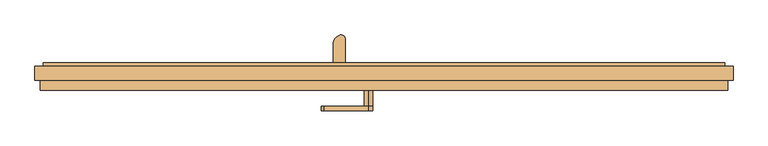
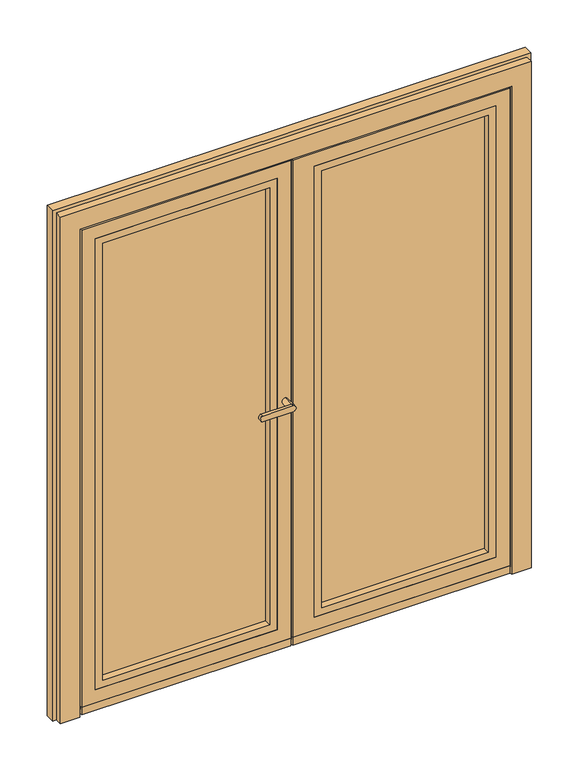
"""IFC4 building model written with IfcOpenShell, lengths in millimetres: door geometry, Schueco_FWS_ADS-75-SimplySmart_out_Family-02 : FWS SI insert unit."""

from ifc_helpers import new_model, si_unit, point, frame, frame_2d, origin, place, context, project, spatial, polyline, circle_curve, ellipse_curve, trimmed, segment, composite_curve, outline, extrude, faceted_brep, source, transform, mapped, element, save
from ifc_brep_helpers import plane_surface, cylinder_surface, extruded_surface, advanced_brep


def door_df799cb0(model_context):
    return source(origin(), model_context, "Body", "SolidModel", [
        faceted_brep([(855.0, -57.5000065, 40.0), (855.0, -57.5000065, 2055.0), (855.0, -66.0002823, 2055.0), (855.0, -66.0002823, 40.0), (-12.5, -66.0002823, 40.0), (-12.5, -57.5000065, 40.0), (6.5, -57.5000065, 40.0), (868.0, -57.5000065, 27.0), (868.0, -57.5000065, 2068.0), (6.5, -57.5000065, 2068.0), (6.5, -57.5000065, 2055.0), (6.5, -57.5000065, 27.0), (-12.5, -66.0002823, 2055.0), (74.5, -66.0002823, 95.0), (74.5, -66.0002823, 2000.0), (800.0, -66.0002823, 2000.0), (800.0, -66.0002823, 95.0), (800.0, 0.4997603, 2000.0), (800.0, 0.4997603, 95.0), (74.5, 0.4997603, 95.0), (74.5, 0.4997603, 2000.0), (106.5, 0.4997603, 127.0), (106.5, 0.4997603, 1968.0), (768.0, 0.4997603, 1968.0), (768.0, 0.4997603, 127.0), (768.0, 8.9997177, 1968.0), (768.0, 8.9997177, 127.0), (106.5, 8.9997177, 127.0), (106.5, 8.9997177, 1968.0), (886.9981585, 8.9997177, 8.0018415), (19.5018415, 8.9997177, 8.0018415), (19.5018415, 8.9997177, 2086.9981585), (886.9981585, 8.9997177, 2086.9981585), (886.9981585, 0.4997603, 2086.9981585), (886.9981585, 0.4997603, 8.0018415), (19.5018415, 0.4997603, 8.0018415), (19.5018415, 0.4997603, 2086.9981585), (19.5018415, 0.4997603, 2068.0), (868.0, 0.4997603, 2068.0), (868.0, 0.4997603, 27.0), (19.5018415, 0.4997603, 27.0), (6.5, 0.4997603, 27.0), (6.5, 0.4997603, 2068.0), (-12.5, -57.5000065, 2055.0)], [[[0, 1, 2, 3]], [[3, 4, 5, 6, 0]], [[7, 8, 9, 10, 1, 0, 6, 11]], [[12, 4, 3, 2], [13, 14, 15, 16]], [[16, 15, 17, 18]], [[18, 19, 13, 16]], [[19, 20, 14, 13]], [[18, 17, 20, 19], [21, 22, 23, 24]], [[24, 23, 25, 26]], [[26, 27, 21, 24]], [[27, 28, 22, 21]], [[29, 30, 31, 32], [26, 25, 28, 27]], [[29, 32, 33, 34]], [[34, 35, 30, 29]], [[33, 36, 37, 38, 39, 40, 35, 34]], [[39, 38, 8, 7]], [[7, 11, 41, 40, 39]], [[11, 6, 10, 9, 42, 41]], [[1, 10, 43, 12, 2]], [[20, 17, 15, 14]], [[28, 25, 23, 22]], [[32, 31, 36, 33]], [[9, 8, 38, 37, 42]], [[43, 10, 6, 5]], [[4, 12, 43, 5]], [[37, 36, 31, 30, 35, 40]], [[40, 41, 42, 37]]]),
        extrude(outline(polyline([(95.0, 74.5), (95.0, 800.0), (2000.0, 800.0), (2000.0, 74.5), (95.0, 74.5)]), holes=[polyline([(125.0, 770.0), (125.0, 104.5), (1970.0, 104.5), (1970.0, 770.0), (125.0, 770.0)])]), frame((0.0, -66.0002823, 0.0), z_axis=(0.0, 1.0, 0.0), x_axis=(0.0, 0.0, 1.0)), (0.0, 0.0, 1.0), 28.5000426),
        extrude(outline(polyline([(74.5, -37.5002397), (74.5, 0.4997603), (800.0, 0.4997603), (800.0, -37.5002397), (74.5, -37.5002397)])), frame((0.0, 0.0, 95.0), z_axis=(0.0, 0.0, 1.0), x_axis=(1.0, 0.0, 0.0)), (0.0, 0.0, 1.0), 1905.0),
        extrude(outline(polyline([(855.0, -65.999964), (-12.5, -65.999964), (-12.5, -57.5000065), (855.0, -57.5000065), (855.0, -65.999964)])), frame((0.0, 0.0, 8.0), z_axis=(0.0, 0.0, 1.0), x_axis=(1.0, 0.0, 0.0)), (0.0, 0.0, 1.0), 32.0),
        extrude(outline(composite_curve([segment(polyline([(-17.8439358, 27.0), (-17.8439358, 4.210912)]), True, "CONTINUOUS"), segment(trimmed(circle_curve(frame_2d((-28.496302, 15.2706996)), 15.3555139), [point((-17.8439358, 4.210912))], [point((-39.1486683, 4.210912))], False, "CARTESIAN"), True, "CONTINUOUS"), segment(polyline([(-39.1486683, 4.210912), (-39.1486683, 27.0), (-17.8439358, 27.0)]), True, "CONTINUOUS")], self_intersect=False)), frame((6.5, 0.0, 0.0), z_axis=(1.0, 0.0, 0.0), x_axis=(0.0, 1.0, 0.0)), (0.0, 0.0, 1.0), 861.5),
        extrude(outline(composite_curve([segment(polyline([(-139.1673236, 8.9997177), (-139.1673236, 59.1618682)]), True, "CONTINUOUS"), segment(trimmed(circle_curve(frame_2d((-111.9889059, 59.1618682)), 27.1784177), [point((-139.1673236, 59.1618682))], [point((-121.5260015, 84.6120194))], False, "CARTESIAN"), True, "CONTINUOUS"), segment(trimmed(circle_curve(frame_2d((-117.4485005, 73.7310321)), 11.6198924), [point((-121.5260015, 84.6120194))], [point((-105.8286081, 73.7310321))], False, "CARTESIAN"), True, "CONTINUOUS"), segment(polyline([(-105.8286081, 73.7310321), (-105.8286081, 8.9997177), (-139.1673236, 8.9997177)]), True, "CONTINUOUS")], self_intersect=False)), frame((0.0, 0.0, 2030.9340013), z_axis=(0.0, 0.0, 1.0), x_axis=(1.0, 0.0, 0.0)), (0.0, 0.0, 1.0), 4.0),
        extrude(outline(polyline([(-139.1673236, 12.9997177), (-105.8286081, 12.9997177), (-105.8286081, 8.9997177), (-139.1673236, 8.9997177), (-139.1673236, 12.9997177)])), frame((0.0, 0.0, 2000.9340013), z_axis=(0.0, 0.0, 1.0), x_axis=(1.0, 0.0, 0.0)), (0.0, 0.0, 1.0), 30.0),
        extrude(outline(polyline([(-139.1673236, 12.9997177), (-105.8286081, 12.9997177), (-105.8286081, 8.9997177), (-139.1673236, 8.9997177), (-139.1673236, 12.9997177)])), frame((0.0, 0.0, 56.9340013), z_axis=(0.0, 0.0, 1.0), x_axis=(1.0, 0.0, 0.0)), (0.0, 0.0, 1.0), 30.0),
        extrude(outline(composite_curve([segment(polyline([(-139.1673236, 8.9997177), (-139.1673236, 59.1618682)]), True, "CONTINUOUS"), segment(trimmed(circle_curve(frame_2d((-111.9889059, 59.1618682)), 27.1784177), [point((-139.1673236, 59.1618682))], [point((-121.5260015, 84.6120194))], False, "CARTESIAN"), True, "CONTINUOUS"), segment(trimmed(circle_curve(frame_2d((-117.4485005, 73.7310321)), 11.6198924), [point((-121.5260015, 84.6120194))], [point((-105.8286081, 73.7310321))], False, "CARTESIAN"), True, "CONTINUOUS"), segment(polyline([(-105.8286081, 73.7310321), (-105.8286081, 8.9997177), (-139.1673236, 8.9997177)]), True, "CONTINUOUS")], self_intersect=False)), frame((0.0, 0.0, 52.9340013), z_axis=(0.0, 0.0, 1.0), x_axis=(1.0, 0.0, 0.0)), (0.0, 0.0, 1.0), 4.0),
        advanced_brep(
        [(-109.782924, 57.5977179, 2030.9340013), (-135.217076, 72.2821425, 2030.9340013), (-109.782924, 57.5977179, 56.9340013), (-135.217076, 72.2821425, 56.9340013)],
        [
            (0, 1, ellipse_curve(frame((-122.5, 64.9399302, 2030.9340013), z_axis=(0.0, 0.0, 1.0000000000000002), x_axis=(0.5000002582658958, 0.866025254674503, 0.0)), 21.5840887, 14.6844171)),
            (1, 0, ellipse_curve(frame((-122.5, 64.9399302, 2030.9340013), z_axis=(0.0, 0.0, 1.0000000000000002), x_axis=(0.5000002582658958, 0.866025254674503, 0.0)), 21.5840887, 14.6844171)),
            (2, 3, ellipse_curve(frame((-122.5, 64.9399302, 56.9340013), z_axis=(0.0, 0.0, -1.0000000000000002), x_axis=(-0.866025254674503, 0.5000002582658958, 0.0)), 14.6844171, 21.5840887)),
            (3, 2, ellipse_curve(frame((-122.5, 64.9399302, 56.9340013), z_axis=(0.0, 0.0, -1.0000000000000002), x_axis=(-0.866025254674503, 0.5000002582658958, 0.0)), 14.6844171, 21.5840887)),
            (0, 2),
            (3, 1),
        ],
        [
            plane_surface(frame((-135.217076, 72.2821425, 2030.9340013), z_axis=(0.0, 0.0, 1.0000000000000002), x_axis=(0.5000002582658958, 0.866025254674503, 0.0))),
            plane_surface(frame((-135.217076, 72.2821425, 56.9340013), z_axis=(0.0, 0.0, -1.0000000000000002), x_axis=(-0.5000002582658958, -0.866025254674503, 0.0))),
            extruded_surface(trimmed(ellipse_curve(frame((-122.5, 64.9399302, 56.9340013), z_axis=(0.0, 0.0, -1.0000000000000002), x_axis=(-0.866025254674503, 0.5000002582658958, 0.0)), 14.6844171, 21.5840887), [point((-135.217076, 72.2821425, 56.9340013))], [point((-109.782924, 57.5977179, 56.9340013))], True, "CARTESIAN"), (0.0, 0.0, -1974.0), 1974.0),
            extruded_surface(trimmed(ellipse_curve(frame((-122.5, 64.9399302, 56.9340013), z_axis=(0.0, 0.0, -1.0000000000000002), x_axis=(-0.866025254674503, 0.5000002582658958, 0.0)), 14.6844171, 21.5840887), [point((-109.782924, 57.5977179, 56.9340013))], [point((-135.217076, 72.2821425, 56.9340013))], True, "CARTESIAN"), (0.0, 0.0, -1974.0), 1974.0),
        ],
        [
            (0, [[1, 2]]),
            (1, [[3, 4]]),
            (2, [[5, -4, 6, -1]]),
            (3, [[-6, -3, -5, -2]]),
        ],
    ),
        advanced_brep(
        [(-42.5, -122.0002518, 1038.0113692), (-42.5, -122.0002518, 1061.9886308), (-164.1617926, -122.0002518, 1061.9886308), (-164.1617926, -122.0002518, 1038.0113692), (-42.5, -109.5001648, 1061.9886308), (-42.5, -109.5001648, 1038.0113692), (-164.1617926, -109.5001648, 1038.0113692), (-164.1617926, -109.5001648, 1061.9886308), (-42.5, -66.0002823, 1038.0113692), (-42.5, -66.0002823, 1061.9886308)],
        [
            (0, 1, circle_curve(frame((-42.5, -122.0002518, 1050.0), z_axis=(0.0, -1.0, 0.0), x_axis=(0.0, 0.0, 1.0)), 11.9886308)),
            (1, 2),
            (2, 3, ellipse_curve(frame((-164.1617926, -122.0002518, 1050.0), z_axis=(0.0, -1.0, 0.0), x_axis=(0.0, 0.0, -1.0)), 11.9886308, 7.9050795)),
            (3, 0),
            (4, 5, circle_curve(frame((-42.5, -109.5001648, 1050.0), z_axis=(0.0, -1.0, 0.0), x_axis=(0.0, 0.0, 1.0)), 11.9886308)),
            (5, 6),
            (6, 7, ellipse_curve(frame((-164.1617926, -109.5001648, 1050.0), z_axis=(0.0, 1.0, 0.0), x_axis=(0.0, 0.0, -1.0)), 11.9886308, 7.9050795)),
            (7, 4),
            (3, 6),
            (5, 0),
            (2, 7),
            (1, 4),
            (5, 4, circle_curve(frame((-42.5, -109.5001648, 1050.0), z_axis=(0.0, -1.0, 0.0), x_axis=(0.0, 0.0, 1.0)), 11.9886308)),
            (8, 9, circle_curve(frame((-42.5, -66.0002823, 1050.0), z_axis=(0.0, 1.0, 0.0), x_axis=(0.0, 0.0, 1.0)), 11.9886308)),
            (9, 8, circle_curve(frame((-42.5, -66.0002823, 1050.0), z_axis=(0.0, 1.0, 0.0), x_axis=(0.0, 0.0, 1.0)), 11.9886308)),
            (8, 5),
            (4, 9),
        ],
        [
            plane_surface(frame((-164.1617926, -122.0002518, 1038.0113692), z_axis=(0.0, -1.0, 0.0), x_axis=(-1.0, 0.0, 0.0))),
            plane_surface(frame((-164.1617926, -109.5001648, 1038.0113692), z_axis=(0.0, 1.0, 0.0), x_axis=(1.0, 0.0, 0.0))),
            plane_surface(frame((-42.5, -122.0002518, 1038.0113692), z_axis=(0.0, 0.0, -1.0), x_axis=(0.0, 1.0, 0.0))),
            extruded_surface(trimmed(ellipse_curve(frame((-164.1617926, -109.5001648, 1050.0), z_axis=(0.0, 1.0, 0.0), x_axis=(0.0, 0.0, -1.0)), 11.9886308, 7.9050795), [point((-164.1617926, -109.5001648, 1038.0113692))], [point((-164.1617926, -109.5001648, 1061.9886308))], True, "CARTESIAN"), (0.0, 12.500086999999994, 0.0), 12.500086999999994),
            plane_surface(frame((-164.1617926, -122.0002518, 1061.9886308), z_axis=(0.0, 0.0, 1.0), x_axis=(0.0, 1.0, 0.0))),
            cylinder_surface(frame((-42.5, -109.5001648, 1050.0), z_axis=(0.0, -1.0, 0.0), x_axis=(0.0, 0.0, 1.0)), 11.9886308),
            plane_surface(frame((-42.5, -66.0002823, 1061.9886308), z_axis=(0.0, 1.0, 0.0), x_axis=(-1.0, 0.0, 0.0))),
            cylinder_surface(frame((-42.5, -66.0002823, 1050.0), z_axis=(0.0, -1.0, 0.0), x_axis=(0.0, 0.0, 1.0)), 11.9886308),
        ],
        [
            (0, [[1, 2, 3, 4]]),
            (1, [[5, 6, 7, 8]]),
            (2, [[9, -6, 10, -4]]),
            (3, [[11, -7, -9, -3]]),
            (4, [[12, -8, -11, -2]]),
            (5, [[-10, 13, -12, -1]]),
            (6, [[14, 15]]),
            (7, [[16, -5, 17, -14]]),
            (7, [[-17, -13, -16, -15]]),
        ],
    ),
        faceted_brep([(-855.0, -57.5000065, 40.0), (-855.0, -66.0002823, 40.0), (-855.0, -66.0002823, 2055.0), (-855.0, -57.5000065, 2055.0), (-21.5, -57.5000065, 40.0), (-19.5, -57.5000065, 40.0), (-19.5, -66.0002823, 40.0), (-21.5, -66.0002823, 40.0), (-868.0, -57.5000065, 27.0), (-6.5, -57.5000065, 27.0), (-6.5, -57.5000065, 2068.0), (-868.0, -57.5000065, 2068.0), (-19.5, -57.5000065, 2055.0), (-21.5, -57.5000065, 2055.0), (-19.5, -66.0002823, 2055.0), (-21.5, -66.0002823, 2055.0), (-74.5, -66.0002823, 95.0), (-800.0, -66.0002823, 95.0), (-800.0, -66.0002823, 2000.0), (-74.5, -66.0002823, 2000.0), (-800.0, 0.4997603, 95.0), (-800.0, 0.4997603, 2000.0), (-74.5, 0.4997603, 95.0), (-74.5, 0.4997603, 2000.0), (-106.5, 0.4997603, 127.0), (-768.0, 0.4997603, 127.0), (-768.0, 0.4997603, 1968.0), (-106.5, 0.4997603, 1968.0), (-768.0, 8.9997177, 127.0), (-768.0, 8.9997177, 1968.0), (-106.5, 8.9997177, 127.0), (-106.5, 8.9997177, 1968.0), (12.4981585, 8.9997177, 8.0018415), (-886.9981585, 8.9997177, 8.0018415), (-886.9981585, 8.9997177, 2086.9981585), (12.4981585, 8.9997177, 2086.9981585), (-886.9981585, 0.4997603, 8.0018415), (-886.9981585, 0.4997603, 2086.9981585), (12.4981585, 0.4997603, 8.0018415), (12.4981585, 0.4997603, 2086.9981585), (-6.5, 0.4997603, 27.0), (-868.0, 0.4997603, 27.0), (-868.0, 0.4997603, 2068.0), (-6.5, 0.4997603, 2068.0)], [[[0, 1, 2, 3]], [[1, 0, 4, 5, 6, 7]], [[8, 9, 10, 11], [12, 5, 4, 0, 3, 13]], [[6, 5, 12, 14]], [[6, 14, 15, 2, 1, 7], [16, 17, 18, 19]], [[17, 20, 21, 18]], [[20, 17, 16, 22]], [[22, 16, 19, 23]], [[20, 22, 23, 21], [24, 25, 26, 27]], [[25, 28, 29, 26]], [[28, 25, 24, 30]], [[30, 24, 27, 31]], [[32, 33, 34, 35], [28, 30, 31, 29]], [[33, 36, 37, 34]], [[36, 33, 32, 38]], [[38, 32, 35, 39]], [[36, 38, 39, 37], [40, 41, 42, 43]], [[41, 8, 11, 42]], [[8, 41, 40, 9]], [[9, 40, 43, 10]], [[14, 12, 13, 3, 2, 15]], [[23, 19, 18, 21]], [[31, 27, 26, 29]], [[39, 35, 34, 37]], [[10, 43, 42, 11]]]),
        extrude(outline(polyline([(95.0, -74.5), (2000.0, -74.5), (2000.0, -800.0), (95.0, -800.0), (95.0, -74.5)]), holes=[polyline([(125.0, -770.0), (1970.0, -770.0), (1970.0, -104.5), (125.0, -104.5), (125.0, -770.0)])]), frame((0.0, -66.0002823, 0.0), z_axis=(0.0, 1.0, 0.0), x_axis=(0.0, 0.0, 1.0)), (0.0, 0.0, 1.0), 28.5000426),
        extrude(outline(polyline([(-74.5, -37.5002397), (-800.0, -37.5002397), (-800.0, 0.4997603), (-74.5, 0.4997603), (-74.5, -37.5002397)])), frame((0.0, 0.0, 95.0), z_axis=(0.0, 0.0, 1.0), x_axis=(1.0, 0.0, 0.0)), (0.0, 0.0, 1.0), 1905.0),
        extrude(outline(polyline([(-855.0, -65.999964), (-855.0, -57.5000065), (-19.5, -57.5000065), (-19.5, -65.999964), (-855.0, -65.999964)])), frame((0.0, 0.0, 8.0), z_axis=(0.0, 0.0, 1.0), x_axis=(1.0, 0.0, 0.0)), (0.0, 0.0, 1.0), 32.0),
        extrude(outline(composite_curve([segment(polyline([(-17.8439358, 27.0), (-17.8439358, 4.210912)]), True, "CONTINUOUS"), segment(trimmed(circle_curve(frame_2d((-28.496302, 15.2706996)), 15.3555139), [point((-17.8439358, 4.210912))], [point((-39.1486683, 4.210912))], False, "CARTESIAN"), True, "CONTINUOUS"), segment(polyline([(-39.1486683, 4.210912), (-39.1486683, 27.0), (-17.8439358, 27.0)]), True, "CONTINUOUS")], self_intersect=False)), frame((-868.0, 0.0, 0.0), z_axis=(1.0, 0.0, 0.0), x_axis=(0.0, 1.0, 0.0)), (0.0, 0.0, 1.0), 861.5),
        faceted_brep([(930.999943, 8.9997177, 2130.999943), (930.999943, 0.0, 2130.999943), (930.999943, 0.0, 0.0), (930.999943, 8.9997177, 0.0), (-954.0, 0.0, 0.0), (-954.0, 0.0, 2154.0), (954.0, 0.0, 2154.0), (954.0, 0.0, 0.0), (-930.999943, 0.0, 2130.999943), (-930.999943, 0.0, 0.0), (954.0, -38.0, 0.0), (940.0, -38.0, 0.0), (940.0, -66.0002823, 0.0), (861.9999732, -66.0002823, 0.0), (861.9999732, -57.5000065, 0.0), (882.4999732, -57.5000065, 0.0), (882.4999732, 0.4997603, 0.0), (893.9999732, 0.4997603, 0.0), (893.9999732, 8.9997177, 0.0), (-893.9999732, 8.9997177, 0.0), (-930.999943, 8.9997177, 0.0), (-930.999943, 8.9997177, 2130.999943), (893.9999732, 8.9997177, 2093.9999732), (-893.9999732, 8.9997177, 2093.9999732), (861.9999732, -66.0002823, 2061.9999732), (861.9999732, -57.5000065, 2061.9999732), (-861.9999732, -57.5000065, 0.0), (-882.4999732, -57.5000065, 0.0), (-882.4999732, -57.5000065, 2082.4999732), (882.4999732, -57.5000065, 2082.4999732), (-861.9999732, -57.5000065, 2061.9999732), (-940.0, -66.0002823, 0.0), (-861.9999732, -66.0002823, 0.0), (-861.9999732, -66.0002823, 2061.9999732), (940.0, -66.0002823, 2140.0), (-940.0, -66.0002823, 2140.0), (940.0, -38.0, 2140.0), (-954.0, -38.0, 0.0), (-940.0, -38.0, 0.0), (-940.0, -38.0, 2140.0), (954.0, -38.0, 2154.0), (-954.0, -38.0, 2154.0), (-893.9999732, 0.4997603, 0.0), (-882.4999732, 0.4997603, 0.0), (893.9999732, 0.4997603, 2093.9999732), (-893.9999732, 0.4997603, 2093.9999732), (882.4999732, 0.4997603, 2082.4999732), (-882.4999732, 0.4997603, 2082.4999732)], [[[0, 1, 2, 3]], [[4, 5, 6, 7, 2, 1, 8, 9]], [[3, 2, 7, 10, 11, 12, 13, 14, 15, 16, 17, 18]], [[19, 20, 21, 0, 3, 18, 22, 23]], [[24, 25, 14, 13]], [[26, 27, 28, 29, 15, 14, 25, 30]], [[31, 32, 33, 24, 13, 12, 34, 35]], [[34, 12, 11, 36]], [[37, 38, 39, 36, 11, 10, 40, 41]], [[4, 9, 20, 19, 42, 43, 27, 26, 32, 31, 38, 37]], [[20, 9, 8, 21]], [[18, 17, 44, 22]], [[42, 19, 23, 45]], [[32, 26, 30, 33]], [[31, 35, 39, 38]], [[4, 37, 41, 5]], [[6, 40, 10, 7]], [[43, 42, 45, 44, 17, 16, 46, 47]], [[16, 15, 29, 46]], [[27, 43, 47, 28]], [[21, 8, 1, 0]], [[33, 30, 25, 24]], [[35, 34, 36, 39]], [[23, 22, 44, 45]], [[5, 41, 40, 6]], [[47, 46, 29, 28]]]),
    ])


if __name__ == "__main__":
    model = new_model("IFC4")
    model_context = context("Model", 3, world=origin())
    ifc_project = project(units=[si_unit("LENGTHUNIT", "METRE", prefix="MILLI")], contexts=[model_context])
    site = spatial("IfcSite", under=ifc_project)
    building = spatial("IfcBuilding", under=site)
    placement = place(None, origin())
    door_shape = door_df799cb0(model_context)
    element("IfcDoor", 1, ObjectType="Schueco_FWS_ADS-75-SimplySmart_out_Family-02 : FWS SI insert unit", at=placement, inside=building, context=model_context, shape_type="MappedRepresentation", body=[
        mapped(door_shape, transform((0.0, 0.0, 0.0), x_axis=(1.0, 0.0, 0.0), y_axis=(0.0, 1.0, 0.0), z_axis=(0.0, 0.0, 1.0))),
    ])
    save(model, "model.ifc")

# Revit data of these elements
# Type "Schueco_FWS_ADS-75-SimplySmart_out_Family-02 : FWS SI insert unit"
#   Type Mark = "56"
#   __NOTE__ = "Data describes the optimum values of the entire system. The properites of a selected design option have to be determined on an individual basis!"
#   Wind load resistance = "Class C3"
#   Watertightness = "Class E750"
#   Thermal insulation = "Uf = 1.6 W/(m²K)"
#   Sound insulation = "..."
#   Schueco thermal insulation standard = "Highly thermally insulated"
#   Opening type = "Outward-opening, Flush-fitted"
#   Model = "Schueco ADS 75 SimplySmart"
#   Mechanical loading = "..."
#   Maximum leaf width in mm = "1400"
#   Maximum leaf weight in kg = "200"
#   Maximum leaf height in mm = "3000"
#   Material = "Aluminium"
#   Long term functionality = "..."
#   Construction Type = "Door, double-leaf, outward-opening"
#   Manufacturer = "Schueco International KG"
#   Glazing data = "Triple glazing 38mm"
#   Façade insert unit = "yes"
#   Family creation date = "08.2017"
#   Description = "Schueco Aluminium Door System (ADS)"
#   Burglar resistance = "Class RC 2"
#   Areas of use = "Public buildings, Residential buildings, Side entrance"
#   Analytic Construction = "<None>"
#   Air permeability = "Class 4"
#   Width [instance default] = 1052.393 mm
#   Leaf opening angle [instance default] = 0.00°
#   IOf_T = 38 mm
#   Height [instance default] = 2117.739 mm
#   Glazing area [instance default] = 0.843522 m²
#   F2_W [instance default] = 526.196 mm
#   F1_W [instance default] = 526.196 mm
#   Distance from bottom to handles [instance default] = 1050 mm
#   Clear opening width [instance default] = 868.393 mm
#   Active leaf width = 1100 mm
#   Standard threshold = no
#   Low level threshold = yes
#   Handles = yes
#   All fields of identical width = yes
#   Glass = none
#   Frame = Alu
#   Fittings = none
# Element 1 (IfcDoor, "Schueco_FWS_ADS-75-SimplySmart_out_Family-02 : FWS SI insert unit")
#   Width = 1908 mm
#   Height = 2154 mm
#   Glazing area = 2.43564 m²
#   F2_W = 954 mm
#   F1_W = 954 mm
#   Clear opening width = 1724 mm
#   Materials on its faces: "Alu", "Glass"
# Materials
#   "Alu": class "Glas", colour RGB 140 140 140, transparency 0
#   "Glass": class "Glass", colour RGB 128 128 255, transparency 0.75, Description = "Soda Lime Glass", Cost = 0
